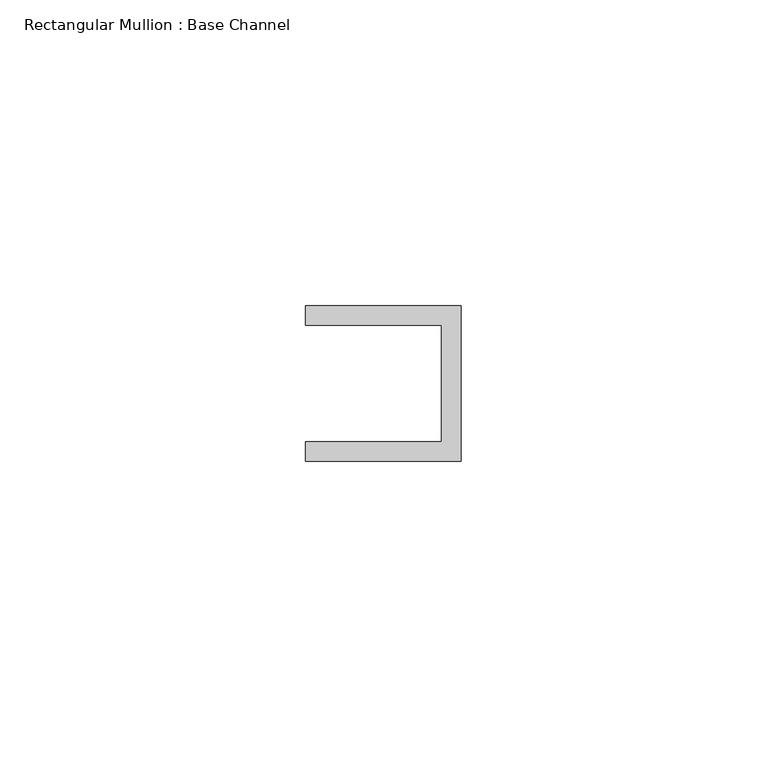
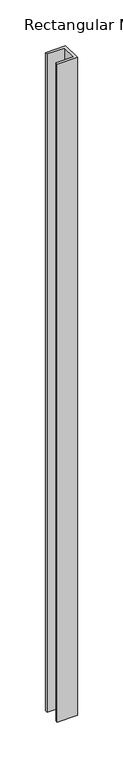
"""IFC4 building model written with IfcOpenShell, lengths in millimetres: member geometry, Rectangular Mullion : Base Channel."""

from ifc_helpers import new_model, si_unit, frame, origin, place, context, project, spatial, polyline, outline, extrude, source, transform, mapped, element, save


def rectangular_mullion_base_channel_30414bef(model_context):
    return source(origin(), model_context, "Body", "SweptSolid", [
        extrude(outline(polyline([(0.0, 12.7), (0.0, -12.7), (-25.4, -12.7), (-25.4, -9.525), (-3.175, -9.525), (-3.175, 9.525), (-25.4, 9.525), (-25.4, 12.7), (0.0, 12.7)])), frame((0.0, 0.0, -876.6174999), z_axis=(0.0, 0.0, 1.0), x_axis=(1.0, 0.0, 0.0)), (0.0, 0.0, 1.0), 876.6174999),
    ])


if __name__ == "__main__":
    model = new_model("IFC4")
    model_context = context("Model", 3, world=origin())
    ifc_project = project(units=[si_unit("LENGTHUNIT", "METRE", prefix="MILLI")], contexts=[model_context])
    site = spatial("IfcSite", under=ifc_project)
    building = spatial("IfcBuilding", under=site)
    placement = place(None, origin())
    rectangular_mullion_base_channel_shape = rectangular_mullion_base_channel_30414bef(model_context)
    element("IfcMember", 1, ObjectType="Rectangular Mullion : Base Channel", at=placement, inside=building, context=model_context, shape_type="MappedRepresentation", body=[
        mapped(rectangular_mullion_base_channel_shape, transform((0.0, 0.0, 0.0), x_axis=(1.0, 0.0, 0.0), y_axis=(0.0, 1.0, 0.0), z_axis=(0.0, 0.0, 1.0))),
    ])
    save(model, "model.ifc")

# Revit data of these elements
# Type "Rectangular Mullion : Base Channel"
#   built-in parameter 1007322 = 0.0833333 (stored number, unit not read)
#   built-in parameter 1007321 = 0.0416667 (stored number, unit not read)
#   built-in parameter 1007320 = -0.03125 (stored number, unit not read)
# Element 1 (IfcMember, "Rectangular Mullion : Base Channel")
#   Materials on its faces: "ALUM"
# Materials
#   "ALUM": class "Generic", colour RGB 157 157 157, transparency 0, Cost = 0
